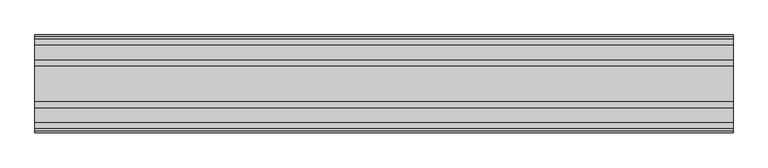
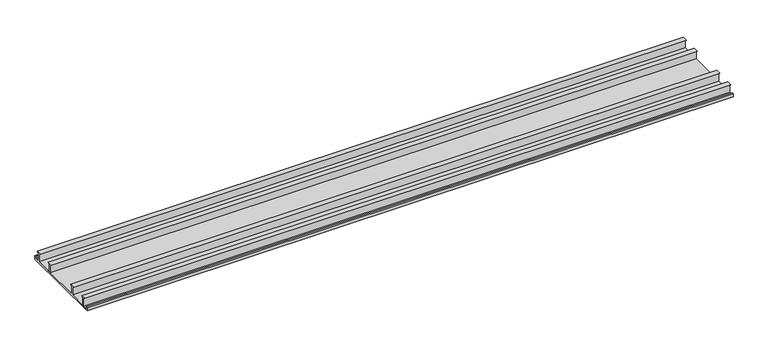
"""IFC4 building model written with IfcOpenShell, lengths in millimetres: proxy geometry, TN_Гидрошпонка ТН Фундамент : Гидрошпонка ТН Фундамент ТШ-Н-210."""

from ifc_helpers import new_model, si_unit, frame, origin, place, context, project, spatial, polyline, outline, extrude, source, transform, mapped, element, save


def specialty_equipment_d27d363f(model_context):
    return source(origin(), model_context, "Body", "SweptSolid", [
        extrude(outline(polyline([(105.0, 0.0), (-105.0, 0.0), (-105.0, 7.9804873), (-102.0, 7.9804873), (-102.0, 4.0), (-92.0456593, 4.0), (-92.0456593, 22.012356), (-96.0, 25.0), (-84.0, 25.0), (-87.9543407, 22.012356), (-87.9543407, 4.0), (-47.0456593, 4.0), (-47.0456593, 22.012356), (-51.0, 25.0), (-39.0, 25.0), (-42.9543407, 22.012356), (-42.9543407, 4.0), (42.9543407, 4.0), (42.9543407, 22.012356), (39.0, 25.0), (51.0, 25.0), (47.0456593, 22.012356), (47.0456593, 4.0), (87.9543407, 4.0), (87.9543407, 22.012356), (84.0, 25.0), (96.0, 25.0), (92.0456593, 22.012356), (92.0456593, 4.0), (102.0, 4.0), (102.0, 7.9804873), (105.0, 7.9804873), (105.0, 0.0)])), frame((0.0, 0.0, 0.0), z_axis=(1.0, 0.0, 0.0), x_axis=(0.0, 1.0, 0.0)), (0.0, 0.0, 1.0), 1500.0),
    ])


if __name__ == "__main__":
    model = new_model("IFC4")
    model_context = context("Model", 3, world=origin())
    ifc_project = project(units=[si_unit("LENGTHUNIT", "METRE", prefix="MILLI")], contexts=[model_context])
    site = spatial("IfcSite", under=ifc_project)
    building = spatial("IfcBuilding", under=site)
    placement = place(None, origin())
    specialty_equipment_shape = specialty_equipment_d27d363f(model_context)
    element("IfcBuildingElementProxy", 1, Name="TN_Гидрошпонка ТН Фундамент : Гидрошпонка ТН Фундамент ТШ-Н-210", ObjectType="TN_Гидрошпонка ТН Фундамент : Гидрошпонка ТН Фундамент ТШ-Н-210", at=placement, inside=building, context=model_context, shape_type="MappedRepresentation", body=[
        mapped(specialty_equipment_shape, transform((0.0, 0.0, 0.0), x_axis=(1.0, 0.0, 0.0), y_axis=(0.0, 1.0, 0.0), z_axis=(0.0, 0.0, 1.0))),
    ])
    save(model, "model.ifc")

# Revit data of these elements
# Type "TN_Гидрошпонка ТН Фундамент : Гидрошпонка ТН Фундамент ТШ-Н-210"
#   Description = "Наружные гидроизоляционные шпонки ТН Фундамент ТШ-Н предназначены для герметизации технологических швов бетонирования при строительстве подземных и заглубленных конструкций зданий и сооружений различного назначения и класса ответственности."
#   Type Comments = "п.м."
#   Manufacturer = "ТехноНИКОЛЬ"
#   URL = "https://nav.tn.ru/catalog/gidroizolyatsiya/komplektatsiya-dlya-gidroizolyatsii/gidroshponki-tekhnonikol-fundament-tsh-n/"
#   ADSK_Примечание = ""
#   ADSK_Обозначение [instance default] = "ТехноНИКОЛЬ"
#   ADSK_Наименование = "Гидрошпонка ТН Фундамент ТШ-Н-210"
#   ADSK_Масса_Текст = ""
#   ADSK_Марка = ""
#   ADSK_Код изделия = "66676"
#   ADSK_Завод-изготовитель [instance default] = "ТехноНИКОЛЬ"
#   ADSK_Единица измерения [instance default] = "п.м."
#   ADSK_Группирование = "Гидрошпонки"
#   ADSK_URL страницы изделия = "https://nav.tn.ru/catalog/gidroizolyatsiya/komplektatsiya-dlya-gidroizolyatsii/gidroshponki-tekhnonikol-fundament-tsh-n/"
#   ADSK_URL документации изделия = "https://nav.tn.ru/upload/iblock/ff2/kxdk1yskynmm632h8p9i264cjgkfwq9e/Tekhlist-7.402_Gidroshponki-TN-Fundament-TSH_N_RU_ru.pdf"
#   built-in parameter 1001306 [instance default] = 3.28084 (stored number, unit not read)
#   ADSK_Размер_Длина [instance default] = 1000 mm
#   ADSK_Количество [instance default] = 1
#   Гидрошпонка ТН Фундамент ТШ-Н-210 = yes
#   Гидрошпонка ТН Фундамент ДШП-В-50 = no
#   Гидрошпонка ТН Фундамент ДШП-В-20 = no
#   Гидрошпонка ТН Фундамент ДШ-В-280 = no
#   Гидрошпонка ТН Фундамент ДШ-В-250 = no
#   Гидрошпонка ТН Фундамент ТШ-В-250 = no
#   Гидрошпонка ТН Фундамент ТПС-В 140-1 = no
#   Гидрошпонка ТН Фундамент ДШ-Н-280 = no
#   Гидрошпонка ТН Фундамент ДШ-Н-250 = no
#   Гидрошпонка ТН Фундамент ТПС-В 100-2 = no
#   Гидрошпонка ТН Фундамент ТШ-Н-250 = no
#   Гидрошпонка ТН Фундамент ТШ-В-210 = no
#   Материал = TN_ПВХ_Черный
#   Default Elevation = 0
# Element 1 (IfcBuildingElementProxy, "TN_Гидрошпонка ТН Фундамент : Гидрошпонка ТН Фундамент ТШ-Н-210")
#   built-in parameter 1001306 = 4.92126 (stored number, unit not read)
#   ADSK_Размер_Длина = 1500 mm
#   ADSK_Количество = 1.5
#   Materials on its faces: "TN_ПВХ_Черный"
# Materials
#   "TN_ПВХ_Черный": class "Типовые", colour RGB 48 48 48, transparency 0, Cost = 0
